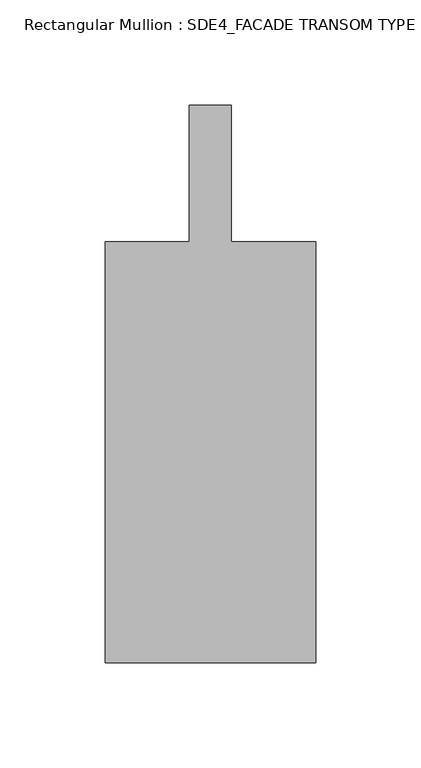
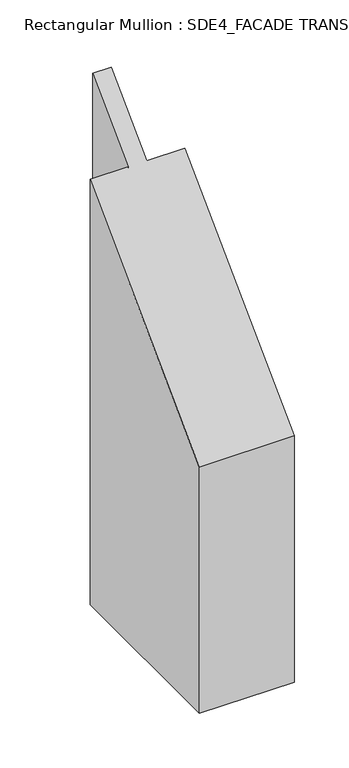
"""IFC4 building model written with IfcOpenShell, lengths in millimetres: member geometry, Rectangular Mullion : SDE4_FACADE TRANSOM TYPE 2."""

from ifc_helpers import new_model, si_unit, origin, place, context, project, spatial, faceted_brep, source, transform, mapped, element, save


def rectangular_mullion_sde4_facade_transom_type_2_39140185(model_context):
    return source(origin(), model_context, "Body", "Brep", [
        faceted_brep([(50.0, -132.5, -407.5), (-50.0, -132.5, -407.5), (-50.0, 67.5, -407.5), (-10.0, 67.5, -407.5), (-10.0, 132.5, -407.5), (10.0, 132.5, -407.5), (10.0, 67.5, -407.5), (50.0, 67.5, -407.5), (50.0, 67.5, 67.5), (50.0, -132.5, -132.5), (10.0, 67.5, 67.5), (10.0, 132.5, 132.5), (-10.0, 132.5, 132.5), (-10.0, 67.5, 67.5), (-50.0, 67.5, 67.5), (-50.0, -132.5, -132.5)], [[[0, 1, 2, 3, 4, 5, 6, 7]], [[8, 9, 0, 7]], [[10, 8, 7, 6]], [[11, 10, 6, 5]], [[12, 11, 5, 4]], [[13, 12, 4, 3]], [[14, 13, 3, 2]], [[15, 14, 2, 1]], [[9, 15, 1, 0]], [[9, 8, 10, 11, 12, 13, 14, 15]]]),
    ])


if __name__ == "__main__":
    model = new_model("IFC4")
    model_context = context("Model", 3, world=origin())
    ifc_project = project(units=[si_unit("LENGTHUNIT", "METRE", prefix="MILLI")], contexts=[model_context])
    site = spatial("IfcSite", under=ifc_project)
    building = spatial("IfcBuilding", under=site)
    placement = place(None, origin())
    rectangular_mullion_sde4_facade_transom_type_2_shape = rectangular_mullion_sde4_facade_transom_type_2_39140185(model_context)
    element("IfcMember", 1, ObjectType="Rectangular Mullion : SDE4_FACADE TRANSOM TYPE 2", at=placement, inside=building, context=model_context, shape_type="MappedRepresentation", body=[
        mapped(rectangular_mullion_sde4_facade_transom_type_2_shape, transform((0.0, 0.0, 0.0), x_axis=(1.0, 0.0, 0.0), y_axis=(0.0, 1.0, 0.0), z_axis=(0.0, 0.0, 1.0))),
    ])
    save(model, "model.ifc")

# Revit data of these elements
# Type "Rectangular Mullion : SDE4_FACADE TRANSOM TYPE 2"
#   built-in parameter 1007322 = 0.869423 (stored number, unit not read)
#   built-in parameter 1007321 = 0.164042 (stored number, unit not read)
#   built-in parameter 1007320 = 0.164042 (stored number, unit not read)
